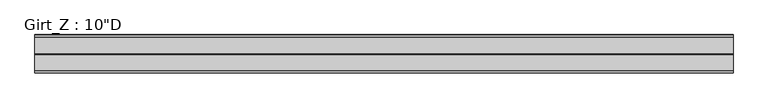
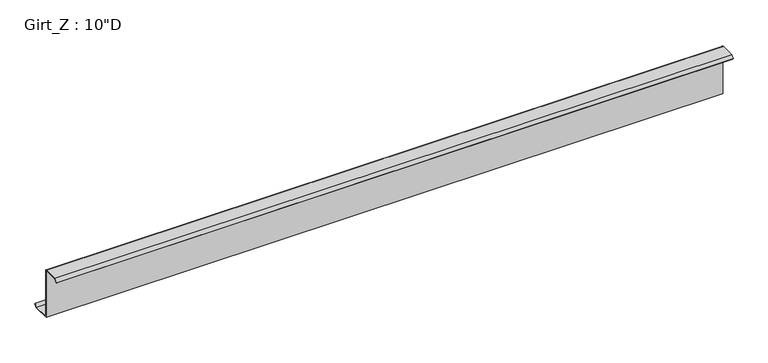
"""IFC4 building model written with IfcOpenShell, lengths in millimetres: beam geometry."""

from ifc_helpers import new_model, si_unit, point, frame, frame_2d, origin, place, context, project, spatial, polyline, circle_curve, trimmed, segment, composite_curve, outline, extrude, source, transform, mapped, element, save


def beam_4a107349(model_context):
    return source(origin(), model_context, "Body", "SweptSolid", [
        extrude(outline(composite_curve([segment(polyline([(-77.9859375, 127.0), (-3.3734375, 127.0)]), True, "CONTINUOUS"), segment(trimmed(circle_curve(frame_2d((-3.3734375, 122.2375)), 4.7625), [point((-3.3734375, 127.0))], [point((1.3890625, 122.2375))], False, "CARTESIAN"), True, "CONTINUOUS"), segment(polyline([(1.3890625, 122.2375), (1.3890625, -122.2389339)]), True, "CONTINUOUS"), segment(trimmed(circle_curve(frame_2d((3.3748024, -122.2389339)), 1.9857399), [point((1.3890625, -122.2389339))], [point((3.2694106, -124.221875))], True, "CARTESIAN"), True, "CONTINUOUS"), segment(polyline([(3.2694106, -124.221875), (83.0404765, -124.221875), (94.4528742, -110.621109), (96.5810415, -112.4068534), (84.3359375, -127.0), (-1.3890625, -127.0), (-1.3890625, 122.2381931)]), True, "CONTINUOUS"), segment(trimmed(circle_curve(frame_2d((-3.3741066, 122.2381931)), 1.9850441), [point((-1.3890625, 122.2381931))], [point((-3.3005807, 124.221875))], True, "CARTESIAN"), True, "CONTINUOUS"), segment(polyline([(-3.3005807, 124.221875), (-76.6904765, 124.221875), (-88.1028742, 110.621109), (-90.2310415, 112.4068534), (-77.9859375, 127.0)]), True, "CONTINUOUS")], self_intersect=False)), frame((-1706.5625, 0.0, 0.0), z_axis=(1.0, 0.0, 0.0), x_axis=(0.0, 1.0, 0.0)), (0.0, 0.0, 1.0), 3403.219),
    ])


if __name__ == "__main__":
    model = new_model("IFC4")
    model_context = context("Model", 3, world=origin())
    ifc_project = project(units=[si_unit("LENGTHUNIT", "METRE", prefix="MILLI")], contexts=[model_context])
    site = spatial("IfcSite", under=ifc_project)
    building = spatial("IfcBuilding", under=site)
    placement = place(None, origin())
    beam_shape = beam_4a107349(model_context)
    element("IfcBeam", 1, ObjectType="Girt_Z : 10\"D", at=placement, inside=building, context=model_context, shape_type="MappedRepresentation", body=[
        mapped(beam_shape, transform((0.0, 0.0, 0.0), x_axis=(1.0, 0.0, 0.0), y_axis=(0.0, 1.0, 0.0), z_axis=(0.0, 0.0, 1.0))),
    ])
    save(model, "model.ifc")

# Revit data of these elements
# Type "Girt_Z : 10\"D"
#   half leg = 0' - 1 11/16"
#   Web_Thickness = 0' - 0 7/64"
#   Length [instance default] = 10' - 0"
#   Leg_2 = 0' - 3 3/8"
#   Leg_1 = 0' - 3 1/8"
#   Height = 0' - 10"
#   Structural Material [instance default] = none
